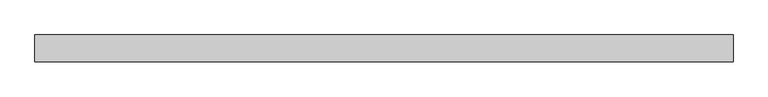
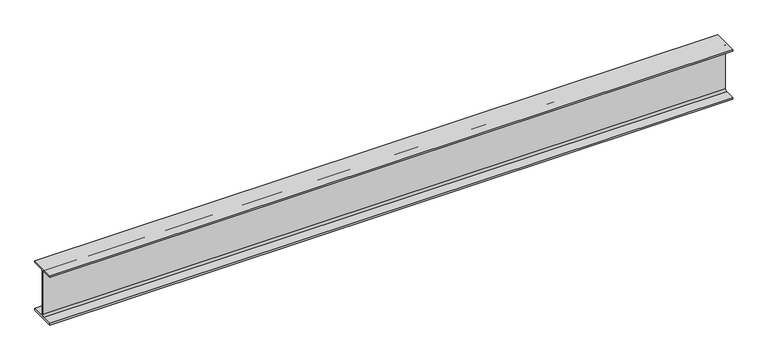
"""IFC4 building model written with IfcOpenShell, lengths in millimetres: beam geometry, 0912_Steel Framing_H-KSD3502 : H_SB_AR_S02_H-350x175x7x11_Platform."""

from ifc_helpers import new_model, si_unit, point, frame, frame_2d, origin, place, context, project, spatial, polyline, circle_curve, trimmed, segment, composite_curve, outline, extrude, source, transform, mapped, element, save


def beam_68894c75(model_context):
    return source(origin(), model_context, "Body", "SweptSolid", [
        extrude(outline(composite_curve([segment(polyline([(87.5, -164.0), (87.5, -175.0), (-87.5, -175.0), (-87.5, -164.0), (-17.5, -164.0)]), True, "CONTINUOUS"), segment(trimmed(circle_curve(frame_2d((-17.5, -150.0)), 14.0), [point((-17.5, -164.0))], [point((-3.5, -150.0))], True, "CARTESIAN"), True, "CONTINUOUS"), segment(polyline([(-3.5, -150.0), (-3.5, 150.0)]), True, "CONTINUOUS"), segment(trimmed(circle_curve(frame_2d((-17.5, 150.0)), 14.0), [point((-3.5, 150.0))], [point((-17.5, 164.0))], True, "CARTESIAN"), True, "CONTINUOUS"), segment(polyline([(-17.5, 164.0), (-87.5, 164.0), (-87.5, 175.0), (87.5, 175.0), (87.5, 164.0), (17.5, 164.0)]), True, "CONTINUOUS"), segment(trimmed(circle_curve(frame_2d((17.5, 150.0)), 14.0), [point((17.5, 164.0))], [point((3.5, 150.0))], True, "CARTESIAN"), True, "CONTINUOUS"), segment(polyline([(3.5, 150.0), (3.5, -150.0)]), True, "CONTINUOUS"), segment(trimmed(circle_curve(frame_2d((17.5, -150.0)), 14.0), [point((3.5, -150.0))], [point((17.5, -164.0))], True, "CARTESIAN"), True, "CONTINUOUS"), segment(polyline([(17.5, -164.0), (87.5, -164.0)]), True, "CONTINUOUS")], self_intersect=False)), frame((-2287.3, 0.0, 0.0), z_axis=(1.0, 0.0, 0.0), x_axis=(0.0, 1.0, 0.0)), (0.0, 0.0, 1.0), 4574.6),
    ])


if __name__ == "__main__":
    model = new_model("IFC4")
    model_context = context("Model", 3, world=origin())
    ifc_project = project(units=[si_unit("LENGTHUNIT", "METRE", prefix="MILLI")], contexts=[model_context])
    site = spatial("IfcSite", under=ifc_project)
    building = spatial("IfcBuilding", under=site)
    placement = place(None, origin())
    beam_shape = beam_68894c75(model_context)
    element("IfcBeam", 1, ObjectType="0912_Steel Framing_H-KSD3502 : H_SB_AR_S02_H-350x175x7x11_Platform", at=placement, inside=building, context=model_context, shape_type="MappedRepresentation", body=[
        mapped(beam_shape, transform((0.0, 0.0, 0.0), x_axis=(1.0, 0.0, 0.0), y_axis=(0.0, 1.0, 0.0), z_axis=(0.0, 0.0, 1.0))),
    ])
    save(model, "model.ifc")

# Revit data of these elements
# Type "0912_Steel Framing_H-KSD3502 : H_SB_AR_S02_H-350x175x7x11_Platform"
#   H_Q'ty Cal Type Tag = "SB-Q2"
#   H_WM Code_1 = "S01AA073-00001 |  | TON | Main Steel Structure Fabrication Work | Shelter/Building | Medium Steel - Standard |  |  |  |  |  |  | Material: (   ) | (90)KG/M>Weight≥(30)KG/M | S01AA073-00001 Main Steel Structure Fabrication Work Shelter/Building Medium Steel - Standard         | - Material: ( ASTM A36 )\n- (90)KG/M>Weight≥(30)KG/M"
#   H_WM Code_2 = "S03AA083-00001 |  | TON | Main Steel Structure Erection Work | Shelter/Building | Medium Steel |  |  |  |  |  |  | Material: (   ) | S03AA083-00001 Main Steel Structure Erection Work Shelter/Building Medium Steel         | - Material: ( ASTM A36 )"
#   H_WM Code_3 = "S01AA009-00001 |  | TON | Main Steel Structure Fabrication Work | Shelter/Building | Plates - Gusset, Stiffener, ETC | Material: (   ) | S01AA009-00001 Main Steel Structure Fabrication Work Shelter/Building Plates - Gusset, Stiffener, ETC         |"
#   H_WM Code_4 = "S41AA051-00001 |  | M2 | Steel Structure Paint Work | Shelter/Building | for Non-Fireproofed Steel Surface |  |  |  |  |  |  | Material: (   ) | S41AA051-00001 Steel Structure Paint Work Shelter/Building for Non-Fireproofed Steel Surface         |"
#   Width = 17.5 cm
#   Web Thickness = 0.7 cm
#   Web Fillet = 1.4 cm
#   Warping Constant = 282000.0 cm⁶
#   W = 0
#   Torsional Moment of Inertia = 19.4042 cm⁴
#   Section Area = 63.14 cm²
#   Plastic Modulus weak axis = 174.0 cm³
#   Plastic Modulus strong axis = 868.0 cm³
#   Perimeter = 1.36 m²/m
#   Nominal Weight = 49.60 kgf/m
#   Moment of Inertia weak axis = 984.00 cm⁴
#   Moment of Inertia strong axis = 13600.00 cm⁴
#   Height = 35.0 cm
#   Flange Thickness = 1.1 cm
#   Elastic Modulus weak axis = 112.0 cm³
#   Elastic Modulus strong axis = 775.0 cm³
#   Centroid Vertical = 17.5 cm
#   Centroid Horizontal = 8.75 cm
#   Ix = 136000000
#   Length [instance default] = 1524 mm
#   Zx = 868000
#   b = 175 mm
#   h = 350 mm
#   r = 14 mm
#   s = 7 mm
#   t = 11 mm
#   A = 0.006314 m²
#   Structural Material [instance default] = Steel, 45-345
#   Assembly Code = ""
# Element 1 (IfcBeam, "0912_Steel Framing_H-KSD3502 : H_SB_AR_S02_H-350x175x7x11_Platform")
#   Materials on its faces: "Steel, 45-345"
# Materials
#   "Steel, 45-345": class "Metal", colour RGB 189 187 185, transparency 0, Description = "Steel 345 MPa", Cost = 0
